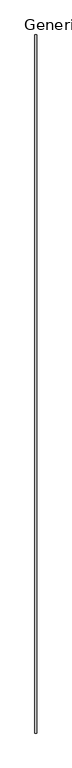
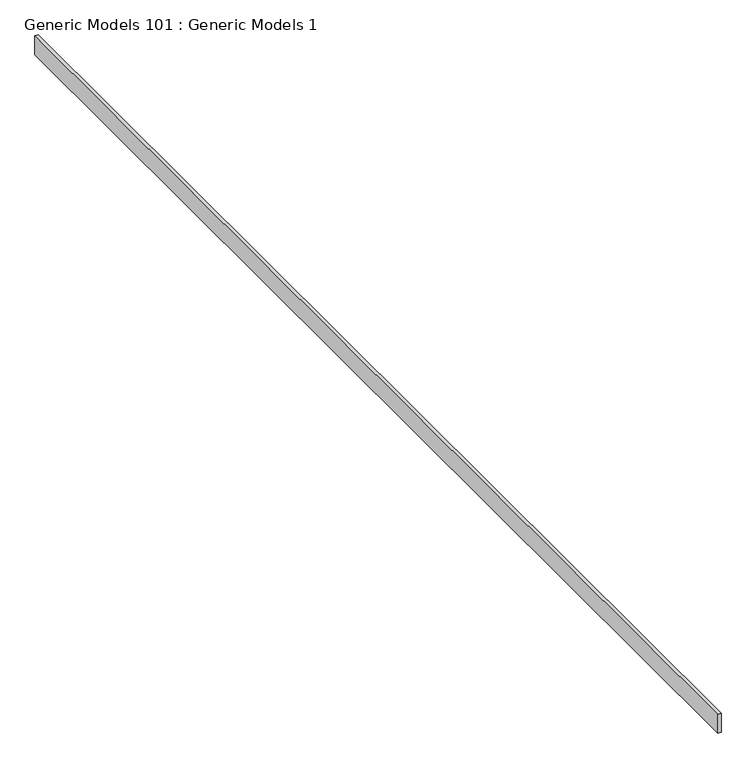
"""IFC4 building model written with IfcOpenShell, lengths in millimetres: proxy geometry, Generic Models 101 : Generic Models 1."""

from ifc_helpers import new_model, si_unit, frame, origin, place, context, project, spatial, polyline, outline, extrude, source, transform, mapped, element, save


def generic_models_101_generic_models_1_afd9d52b(model_context):
    return source(origin(), model_context, "Body", "SweptSolid", [
        extrude(outline(polyline([(-6565.7647071, 7054.2769662), (-6527.6647071, 7054.2769662), (-6527.6647071, -7068.1230338), (-6565.7647071, -7068.1230338), (-6565.7647071, 7054.2769662)])), frame((0.0, 0.0, 126415.927), z_axis=(0.0, 0.0, 1.0), x_axis=(1.0, 0.0, 0.0)), (0.0, 0.0, 1.0), 234.95),
    ])


if __name__ == "__main__":
    model = new_model("IFC4")
    model_context = context("Model", 3, world=origin())
    ifc_project = project(units=[si_unit("LENGTHUNIT", "METRE", prefix="MILLI")], contexts=[model_context])
    site = spatial("IfcSite", under=ifc_project)
    building = spatial("IfcBuilding", under=site)
    placement = place(None, origin())
    generic_models_101_generic_models_1_shape = generic_models_101_generic_models_1_afd9d52b(model_context)
    element("IfcBuildingElementProxy", 1, Name="Generic Models 101 : Generic Models 1", ObjectType="Generic Models 101 : Generic Models 1", at=placement, inside=building, context=model_context, shape_type="MappedRepresentation", body=[
        mapped(generic_models_101_generic_models_1_shape, transform((0.0, 0.0, 0.0), x_axis=(1.0, 0.0, 0.0), y_axis=(0.0, 1.0, 0.0), z_axis=(0.0, 0.0, 1.0))),
    ])
    save(model, "model.ifc")

# Revit data of these elements
# Element 1 (IfcBuildingElementProxy, "Generic Models 101 : Generic Models 1")
#   Materials on its faces: "_2X STRUCTURAL BLOCKING (SEE STRUCT. DWGS)"
# Materials
#   "_2X STRUCTURAL BLOCKING (SEE STRUCT. DWGS)": class "Generic", colour RGB 177 130 114, transparency 0, Cost = 0
